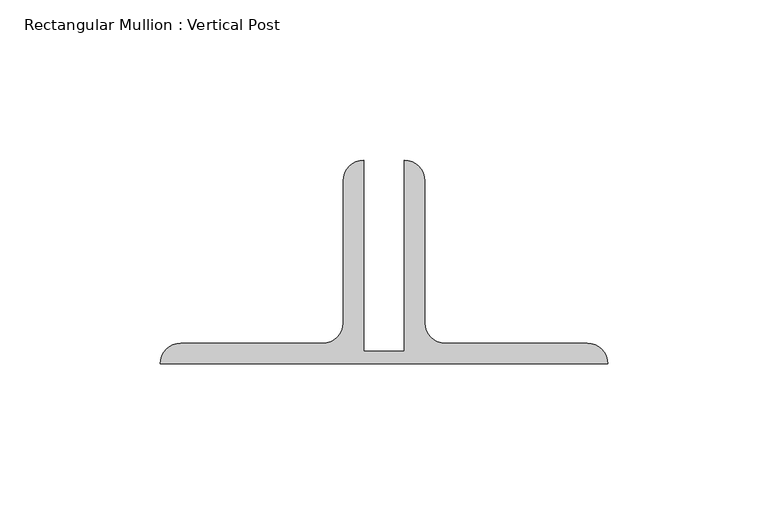
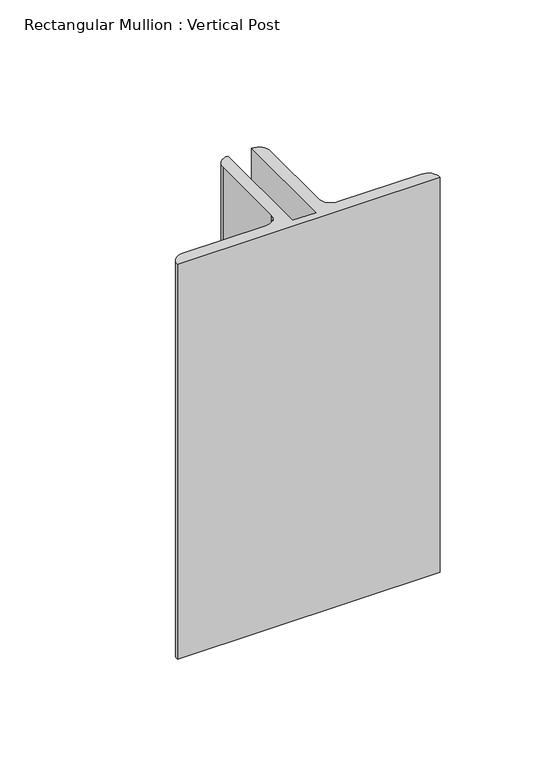
"""IFC4 building model written with IfcOpenShell, lengths in millimetres: member geometry, Rectangular Mullion : Vertical Post."""

import ifcopenshell
import ifcopenshell.guid

model = None  # the IFC model being written
_history = None  # IfcOwnerHistory: only IFC2X3 demands one
_inside = {}  # id of a spatial element -> (the spatial element, [elements in it])
_under = {}  # id of a project, library or spatial element -> (it, [spatial elements below it])
_declared = {}  # id of a project -> (the project, [libraries it declares])
_typed = {}  # id of a type object -> (the type object, [elements of that type])
_made_of = {}  # id of a material, layer set ... -> (it, [elements and type objects made of it])


def new_model(schema):
    """Start an empty IFC model of exactly this schema.

    Asked for "IFC4X3", IfcOpenShell would pick the latest addendum, in which some entities
    have other attributes; the version numbers below select the first issue.
    IFC2X3 requires an IfcOwnerHistory on every rooted entity: one is made here for all.
    """
    global model, _history
    if schema == "IFC4X3":
        model = ifcopenshell.file(schema_version=(4, 3, 0, 0))
    else:
        model = ifcopenshell.file(schema=schema)
    _inside.clear()
    _under.clear()
    _declared.clear()
    _typed.clear()
    _made_of.clear()
    _history = None
    if model.schema == "IFC2X3":
        org = make("IfcOrganization", Name="unknown")
        user = make(
            "IfcPersonAndOrganization",
            ThePerson=make("IfcPerson", FamilyName="unknown"),
            TheOrganization=org,
        )
        app = make(
            "IfcApplication",
            ApplicationDeveloper=org,
            Version="unknown",
            ApplicationFullName="unknown",
            ApplicationIdentifier="unknown",
        )
        _history = make(
            "IfcOwnerHistory",
            OwningUser=user,
            OwningApplication=app,
            ChangeAction="ADDED",
            CreationDate=0,
        )
    return model


def make(cls, **values):
    """One entity of the class cls with the attributes given. An attribute that is None is left unset."""
    return model.create_entity(
        cls, **{name: value for name, value in values.items() if value is not None}
    )


def rooted(cls, **values):
    """An entity with a GlobalId (a new one), such as an element, a storey or a relation."""
    return make(cls, GlobalId=ifcopenshell.guid.new(), OwnerHistory=_history, **values)


def si_unit(unit_type, name, prefix=None):
    """IfcSIUnit, for example si_unit("LENGTHUNIT", "METRE", prefix="MILLI")."""
    return make("IfcSIUnit", UnitType=unit_type, Prefix=prefix, Name=name)


def assignment(units):
    """IfcUnitAssignment: the units of a project."""
    return None if units is None else make("IfcUnitAssignment", Units=units)


def point(xyz):
    """IfcCartesianPoint."""
    return None if xyz is None else make("IfcCartesianPoint", Coordinates=xyz)


def direction(xyz):
    """IfcDirection."""
    return None if xyz is None else make("IfcDirection", DirectionRatios=xyz)


def frame(location, z_axis=None, x_axis=None):
    """IfcAxis2Placement3D, a coordinate frame: its origin and axes. An axis left out is left unset."""
    return make(
        "IfcAxis2Placement3D",
        Location=point(location),
        Axis=direction(z_axis),
        RefDirection=direction(x_axis),
    )


def frame_2d(location, x_axis=None):
    """IfcAxis2Placement2D, a coordinate frame in the plane: its origin and x axis."""
    return make(
        "IfcAxis2Placement2D", Location=point(location), RefDirection=direction(x_axis)
    )


def origin():
    """The frame at (0, 0, 0) with its axes left unset."""
    return frame((0.0, 0.0, 0.0))


def place(relative_to, where):
    """IfcLocalPlacement: puts the frame where relative to a parent placement (None: the world)."""
    return make(
        "IfcLocalPlacement", PlacementRelTo=relative_to, RelativePlacement=where
    )


def context(
    kind, dimensions, precision=None, world=None, true_north=None, identifier=None
):
    """IfcGeometricRepresentationContext, for example the 3D "Model" context."""
    return make(
        "IfcGeometricRepresentationContext",
        ContextIdentifier=identifier,
        ContextType=kind,
        CoordinateSpaceDimension=dimensions,
        Precision=precision,
        WorldCoordinateSystem=world,
        TrueNorth=true_north,
    )


def project(units=None, contexts=None):
    """IfcProject with its units and contexts."""
    return rooted(
        "IfcProject",
        Name="project",
        RepresentationContexts=contexts,
        UnitsInContext=assignment(units),
    )


def spatial(cls, under=None, at=None, **own):
    """A site, building, storey or space (cls), placed at a placement, below another one or the project."""
    s = rooted(cls, ObjectPlacement=at, **own)
    if under is not None:
        _under.setdefault(under.id(), (under, []))[1].append(s)
    return s


def polyline(points):
    """IfcPolyline through the points."""
    return make("IfcPolyline", Points=[point(p) for p in points])


def circle_curve(where, radius):
    """IfcCircle in the frame where."""
    return make("IfcCircle", Position=where, Radius=radius)


def trimmed(basis, trim1, trim2, sense, master):
    """IfcTrimmedCurve: the piece of a basis curve between two trims."""
    return make(
        "IfcTrimmedCurve",
        BasisCurve=basis,
        Trim1=trim1,
        Trim2=trim2,
        SenseAgreement=sense,
        MasterRepresentation=master,
    )


def segment(curve, same_sense, transition):
    """IfcCompositeCurveSegment."""
    return make(
        "IfcCompositeCurveSegment",
        Transition=transition,
        SameSense=same_sense,
        ParentCurve=curve,
    )


def composite_curve(segments, self_intersect=None):
    """IfcCompositeCurve: segments joined end to end."""
    return make("IfcCompositeCurve", Segments=segments, SelfIntersect=self_intersect)


def outline(outer, holes=None, kind="AREA"):
    """IfcArbitraryClosedProfileDef: a profile drawn as a closed curve; with holes, ...WithVoids."""
    if holes is None:
        return make("IfcArbitraryClosedProfileDef", ProfileType=kind, OuterCurve=outer)
    return make(
        "IfcArbitraryProfileDefWithVoids",
        ProfileType=kind,
        OuterCurve=outer,
        InnerCurves=holes,
    )


def extrude(swept, where, along, depth):
    """IfcExtrudedAreaSolid: the profile swept, set in the frame where, extruded along a direction by depth."""
    return make(
        "IfcExtrudedAreaSolid",
        SweptArea=swept,
        Position=where,
        ExtrudedDirection=direction(along),
        Depth=depth,
    )


def shape(context_of_items, identifier, shape_type, items):
    """IfcShapeRepresentation: the items that make up one representation, for example the "Body"."""
    return make(
        "IfcShapeRepresentation",
        ContextOfItems=context_of_items,
        RepresentationIdentifier=identifier,
        RepresentationType=shape_type,
        Items=items,
    )


def source(mapping_origin, context_of_items, identifier, shape_type, items):
    """IfcRepresentationMap: a shape defined once, which mapped items show again and again."""
    return make(
        "IfcRepresentationMap",
        MappingOrigin=mapping_origin,
        MappedRepresentation=shape(context_of_items, identifier, shape_type, items),
    )


def transform(
    local_origin,
    x_axis=None,
    y_axis=None,
    z_axis=None,
    scale=None,
    scale2=None,
    scale3=None,
    uniform=True,
):
    """IfcCartesianTransformationOperator3D, or its non-uniform kind. x_axis, y_axis, z_axis: its Axis1, 2, 3."""
    if uniform:
        return make(
            "IfcCartesianTransformationOperator3D",
            Axis1=direction(x_axis),
            Axis2=direction(y_axis),
            LocalOrigin=point(local_origin),
            Scale=scale,
            Axis3=direction(z_axis),
        )
    return make(
        "IfcCartesianTransformationOperator3DnonUniform",
        Axis1=direction(x_axis),
        Axis2=direction(y_axis),
        LocalOrigin=point(local_origin),
        Scale=scale,
        Axis3=direction(z_axis),
        Scale2=scale2,
        Scale3=scale3,
    )


def mapped(mapping_source, mapping_target):
    """IfcMappedItem: shows the shape of a source again, moved by a transform."""
    return make(
        "IfcMappedItem", MappingSource=mapping_source, MappingTarget=mapping_target
    )


def made_of(thing, what):
    """Note that an element or type object is made of a material, layer set ...; save() writes the relation."""
    if what is not None:
        _made_of.setdefault(what.id(), (what, []))[1].append(thing)
    return thing


def element(
    cls,
    number,
    at=None,
    inside=None,
    cuts=None,
    type_object=None,
    material=None,
    context=None,
    identifier="Body",
    shape_type=None,
    held_by="IfcProductDefinitionShape",
    body=None,
    shapes=None,
    **own,
):
    """One element of the class cls, such as IfcWall. Its Tag is "e" and its number.

    at: its placement. inside: the storey or other place that contains it. cuts: it is an
    opening in that element (IfcRelVoidsElement). A single representation is given by context,
    identifier, shape_type and body (its items); several are given by shapes. held_by: the class
    of the entity that holds the representations. save() writes the other relations.
    """
    e = rooted(cls, Tag="e%d" % number, ObjectPlacement=at, **own)
    if body is not None:
        shapes = [shape(context, identifier, shape_type, body)]
    if shapes is not None:
        e.Representation = make(held_by, Representations=shapes)
    if inside is not None:
        _inside.setdefault(inside.id(), (inside, []))[1].append(e)
    if cuts is not None:
        rooted(
            "IfcRelVoidsElement", RelatingBuildingElement=cuts, RelatedOpeningElement=e
        )
    if type_object is not None:
        _typed.setdefault(type_object.id(), (type_object, []))[1].append(e)
    return made_of(e, material)


def aggregate(whole, parts):
    """IfcRelAggregates: a whole, such as a stair, and the parts it consists of."""
    return rooted("IfcRelAggregates", RelatingObject=whole, RelatedObjects=parts)


def save(model, path):
    """Write the relations noted so far, then the file.

    IfcRelAggregates (storeys below a building ...), IfcRelContainedInSpatialStructure (elements
    in a storey), IfcRelDefinesByType, IfcRelAssociatesMaterial and IfcRelDeclares: one each for
    every whole, place, type object, material and project.
    """
    for whole, parts in _under.values():
        aggregate(whole, parts)
    for where, things in _inside.values():
        rooted(
            "IfcRelContainedInSpatialStructure",
            RelatedElements=things,
            RelatingStructure=where,
        )
    for kind, things in _typed.values():
        rooted("IfcRelDefinesByType", RelatedObjects=things, RelatingType=kind)
    for what, things in _made_of.values():
        rooted("IfcRelAssociatesMaterial", RelatedObjects=things, RelatingMaterial=what)
    for by, libraries in _declared.values():
        rooted("IfcRelDeclares", RelatingContext=by, RelatedDefinitions=libraries)
    model.write(path)


def rectangular_mullion_vertical_post_21cc10da(model_context):
    return source(origin(), model_context, "Body", "SweptSolid", [
        extrude(outline(composite_curve([segment(polyline([(-76.2, 22.9145205), (-63.5, 22.9145205), (-63.5, 82.55)]), True, "CONTINUOUS"), segment(trimmed(circle_curve(frame_2d((-63.5, 76.2)), 6.35), [point((-63.5, 82.55))], [point((-57.15, 76.2))], False, "CARTESIAN"), True, "CONTINUOUS"), segment(polyline([(-57.15, 76.2), (-57.15, 31.75)]), True, "CONTINUOUS"), segment(trimmed(circle_curve(frame_2d((-50.8, 31.75)), 6.35), [point((-57.15, 31.75))], [point((-50.8, 25.4))], True, "CARTESIAN"), True, "CONTINUOUS"), segment(polyline([(-50.8, 25.4), (-6.35, 25.4)]), True, "CONTINUOUS"), segment(trimmed(circle_curve(frame_2d((-6.35, 19.05)), 6.35), [point((-6.35, 25.4))], [point((0.0, 19.05))], False, "CARTESIAN"), True, "CONTINUOUS"), segment(polyline([(0.0, 19.05), (-139.7, 19.05)]), True, "CONTINUOUS"), segment(trimmed(circle_curve(frame_2d((-133.35, 19.05)), 6.35), [point((-139.7, 19.05))], [point((-133.35, 25.4))], False, "CARTESIAN"), True, "CONTINUOUS"), segment(polyline([(-133.35, 25.4), (-88.9, 25.4)]), True, "CONTINUOUS"), segment(trimmed(circle_curve(frame_2d((-88.9, 31.75)), 6.35), [point((-88.9, 25.4))], [point((-82.55, 31.75))], True, "CARTESIAN"), True, "CONTINUOUS"), segment(polyline([(-82.55, 31.75), (-82.55, 76.2)]), True, "CONTINUOUS"), segment(trimmed(circle_curve(frame_2d((-76.2, 76.2)), 6.35), [point((-82.55, 76.2))], [point((-76.2, 82.55))], False, "CARTESIAN"), True, "CONTINUOUS"), segment(polyline([(-76.2, 82.55), (-76.2, 22.9145205)]), True, "CONTINUOUS")], self_intersect=False)), frame((0.0, 0.0, -222.0889998), z_axis=(0.0, 0.0, 1.0), x_axis=(1.0, 0.0, 0.0)), (0.0, 0.0, 1.0), 222.0889998),
    ])


if __name__ == "__main__":
    model = new_model("IFC4")
    model_context = context("Model", 3, world=origin())
    ifc_project = project(units=[si_unit("LENGTHUNIT", "METRE", prefix="MILLI")], contexts=[model_context])
    site = spatial("IfcSite", under=ifc_project)
    building = spatial("IfcBuilding", under=site)
    placement = place(None, origin())
    rectangular_mullion_vertical_post_shape = rectangular_mullion_vertical_post_21cc10da(model_context)
    element("IfcMember", 1, ObjectType="Rectangular Mullion : Vertical Post", at=placement, inside=building, context=model_context, shape_type="MappedRepresentation", body=[
        mapped(rectangular_mullion_vertical_post_shape, transform((0.0, 0.0, 0.0), x_axis=(1.0, 0.0, 0.0), y_axis=(0.0, 1.0, 0.0), z_axis=(0.0, 0.0, 1.0))),
    ])
    save(model, "model.ifc")

# Revit data of these elements
# Type "Rectangular Mullion : Vertical Post"
#   built-in parameter 1007351 = -0.0625 (stored number, unit not read)
#   built-in parameter 1007322 = 0.0126789 (stored number, unit not read)
#   built-in parameter 1007321 = 0.229167 (stored number, unit not read)
#   built-in parameter 1007320 = 0.229167 (stored number, unit not read)
# Element 1 (IfcMember, "Rectangular Mullion : Vertical Post")
#   Materials on its faces: "GATE POST: (2) BACK/BACK GALVANIZED ANGLES"
# Materials
#   "GATE POST: (2) BACK/BACK GALVANIZED ANGLES": class "Unassigned", colour RGB 211 211 211, transparency 0, Cost = 0
